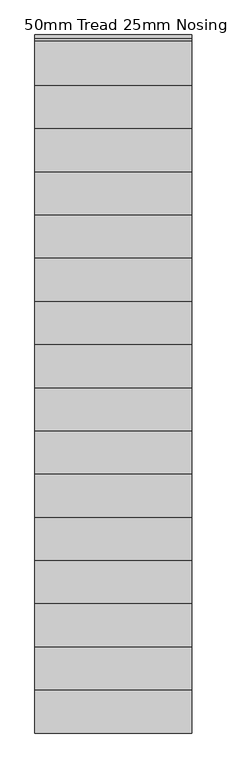
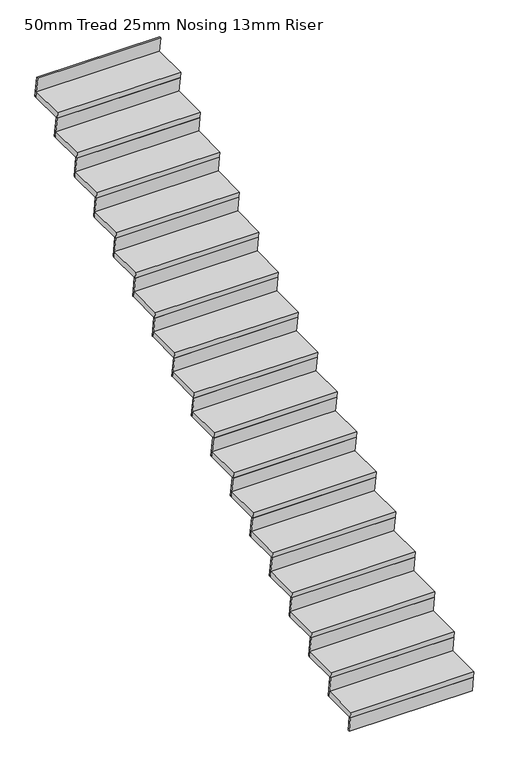
"""IFC4 building model written with IfcOpenShell, lengths in millimetres: stair flight geometry, 50mm Tread 25mm Nosing 13mm Riser."""

from ifc_helpers import new_model, si_unit, frame, origin, place, context, project, spatial, polyline, outline, extrude, source, transform, mapped, element, save


def stair_flight_50mm_tread_25mm_nosing_13mm_riser_3b40119f(model_context):
    return source(origin(), model_context, "Body", "SweptSolid", [
        extrude(outline(polyline([(-31126.6946949, 176.4705882), (-30826.6946949, 176.4705882), (-30819.6113616, 126.4705882), (-31119.6113616, 126.4705882), (-31126.6946949, 176.4705882)])), frame((121318.8827039, 0.0, 0.0), z_axis=(1.0, 0.0, 0.0), x_axis=(0.0, 1.0, 0.0)), (0.0, 0.0, 1.0), 1000.0),
        extrude(outline(polyline([(-31119.6113616, 126.4705882), (-31106.9865507, 126.4705882), (-31089.069884, 0.0), (-31101.6946949, 0.0), (-31119.6113616, 126.4705882)])), frame((121318.8827039, 0.0, 0.0), z_axis=(1.0, 0.0, 0.0), x_axis=(0.0, 1.0, 0.0)), (0.0, 0.0, 1.0), 1000.0),
        extrude(outline(polyline([(-30844.6113616, 302.9411765), (-30831.9865507, 302.9411765), (-30806.9865507, 126.4705882), (-30819.6113616, 126.4705882), (-30844.6113616, 302.9411765)])), frame((121318.8827039, 0.0, 0.0), z_axis=(1.0, 0.0, 0.0), x_axis=(0.0, 1.0, 0.0)), (0.0, 0.0, 1.0), 1000.0),
        extrude(outline(polyline([(-30851.6946949, 352.9411765), (-30551.6946949, 352.9411765), (-30544.6113616, 302.9411765), (-30844.6113616, 302.9411765), (-30851.6946949, 352.9411765)])), frame((121318.8827039, 0.0, 0.0), z_axis=(1.0, 0.0, 0.0), x_axis=(0.0, 1.0, 0.0)), (0.0, 0.0, 1.0), 1000.0),
        extrude(outline(polyline([(-30569.6113616, 479.4117647), (-30556.9865507, 479.4117647), (-30531.9865507, 302.9411765), (-30544.6113616, 302.9411765), (-30569.6113616, 479.4117647)])), frame((121318.8827039, 0.0, 0.0), z_axis=(1.0, 0.0, 0.0), x_axis=(0.0, 1.0, 0.0)), (0.0, 0.0, 1.0), 1000.0),
        extrude(outline(polyline([(-30576.6946949, 529.4117647), (-30276.6946949, 529.4117647), (-30269.6113616, 479.4117647), (-30569.6113616, 479.4117647), (-30576.6946949, 529.4117647)])), frame((121318.8827039, 0.0, 0.0), z_axis=(1.0, 0.0, 0.0), x_axis=(0.0, 1.0, 0.0)), (0.0, 0.0, 1.0), 1000.0),
        extrude(outline(polyline([(-30294.6113616, 655.8823529), (-30281.9865507, 655.8823529), (-30256.9865507, 479.4117647), (-30269.6113616, 479.4117647), (-30294.6113616, 655.8823529)])), frame((121318.8827039, 0.0, 0.0), z_axis=(1.0, 0.0, 0.0), x_axis=(0.0, 1.0, 0.0)), (0.0, 0.0, 1.0), 1000.0),
        extrude(outline(polyline([(-30301.6946949, 705.8823529), (-30001.6946949, 705.8823529), (-29994.6113616, 655.8823529), (-30294.6113616, 655.8823529), (-30301.6946949, 705.8823529)])), frame((121318.8827039, 0.0, 0.0), z_axis=(1.0, 0.0, 0.0), x_axis=(0.0, 1.0, 0.0)), (0.0, 0.0, 1.0), 1000.0),
        extrude(outline(polyline([(-30019.6113616, 832.3529412), (-30006.9865507, 832.3529412), (-29981.9865507, 655.8823529), (-29994.6113616, 655.8823529), (-30019.6113616, 832.3529412)])), frame((121318.8827039, 0.0, 0.0), z_axis=(1.0, 0.0, 0.0), x_axis=(0.0, 1.0, 0.0)), (0.0, 0.0, 1.0), 1000.0),
        extrude(outline(polyline([(-30026.6946949, 882.3529412), (-29726.6946949, 882.3529412), (-29719.6113616, 832.3529412), (-30019.6113616, 832.3529412), (-30026.6946949, 882.3529412)])), frame((121318.8827039, 0.0, 0.0), z_axis=(1.0, 0.0, 0.0), x_axis=(0.0, 1.0, 0.0)), (0.0, 0.0, 1.0), 1000.0),
        extrude(outline(polyline([(-29744.6113616, 1008.8235294), (-29731.9865507, 1008.8235294), (-29706.9865507, 832.3529412), (-29719.6113616, 832.3529412), (-29744.6113616, 1008.8235294)])), frame((121318.8827039, 0.0, 0.0), z_axis=(1.0, 0.0, 0.0), x_axis=(0.0, 1.0, 0.0)), (0.0, 0.0, 1.0), 1000.0),
        extrude(outline(polyline([(-29751.6946949, 1058.8235294), (-29451.6946949, 1058.8235294), (-29444.6113616, 1008.8235294), (-29744.6113616, 1008.8235294), (-29751.6946949, 1058.8235294)])), frame((121318.8827039, 0.0, 0.0), z_axis=(1.0, 0.0, 0.0), x_axis=(0.0, 1.0, 0.0)), (0.0, 0.0, 1.0), 1000.0),
        extrude(outline(polyline([(-29469.6113616, 1185.2941176), (-29456.9865507, 1185.2941176), (-29431.9865507, 1008.8235294), (-29444.6113616, 1008.8235294), (-29469.6113616, 1185.2941176)])), frame((121318.8827039, 0.0, 0.0), z_axis=(1.0, 0.0, 0.0), x_axis=(0.0, 1.0, 0.0)), (0.0, 0.0, 1.0), 1000.0),
        extrude(outline(polyline([(-29476.6946949, 1235.2941176), (-29176.6946949, 1235.2941176), (-29169.6113616, 1185.2941176), (-29469.6113616, 1185.2941176), (-29476.6946949, 1235.2941176)])), frame((121318.8827039, 0.0, 0.0), z_axis=(1.0, 0.0, 0.0), x_axis=(0.0, 1.0, 0.0)), (0.0, 0.0, 1.0), 1000.0),
        extrude(outline(polyline([(-29194.6113616, 1361.7647059), (-29181.9865507, 1361.7647059), (-29156.9865507, 1185.2941176), (-29169.6113616, 1185.2941176), (-29194.6113616, 1361.7647059)])), frame((121318.8827039, 0.0, 0.0), z_axis=(1.0, 0.0, 0.0), x_axis=(0.0, 1.0, 0.0)), (0.0, 0.0, 1.0), 1000.0),
        extrude(outline(polyline([(-29201.6946949, 1411.7647059), (-28901.6946949, 1411.7647059), (-28894.6113616, 1361.7647059), (-29194.6113616, 1361.7647059), (-29201.6946949, 1411.7647059)])), frame((121318.8827039, 0.0, 0.0), z_axis=(1.0, 0.0, 0.0), x_axis=(0.0, 1.0, 0.0)), (0.0, 0.0, 1.0), 1000.0),
        extrude(outline(polyline([(-28919.6113616, 1538.2352941), (-28906.9865507, 1538.2352941), (-28881.9865507, 1361.7647059), (-28894.6113616, 1361.7647059), (-28919.6113616, 1538.2352941)])), frame((121318.8827039, 0.0, 0.0), z_axis=(1.0, 0.0, 0.0), x_axis=(0.0, 1.0, 0.0)), (0.0, 0.0, 1.0), 1000.0),
        extrude(outline(polyline([(-28926.6946949, 1588.2352941), (-28626.6946949, 1588.2352941), (-28619.6113616, 1538.2352941), (-28919.6113616, 1538.2352941), (-28926.6946949, 1588.2352941)])), frame((121318.8827039, 0.0, 0.0), z_axis=(1.0, 0.0, 0.0), x_axis=(0.0, 1.0, 0.0)), (0.0, 0.0, 1.0), 1000.0),
        extrude(outline(polyline([(-28644.6113616, 1714.7058824), (-28631.9865507, 1714.7058824), (-28606.9865507, 1538.2352941), (-28619.6113616, 1538.2352941), (-28644.6113616, 1714.7058824)])), frame((121318.8827039, 0.0, 0.0), z_axis=(1.0, 0.0, 0.0), x_axis=(0.0, 1.0, 0.0)), (0.0, 0.0, 1.0), 1000.0),
        extrude(outline(polyline([(-28651.6946949, 1764.7058824), (-28351.6946949, 1764.7058824), (-28344.6113616, 1714.7058824), (-28644.6113616, 1714.7058824), (-28651.6946949, 1764.7058824)])), frame((121318.8827039, 0.0, 0.0), z_axis=(1.0, 0.0, 0.0), x_axis=(0.0, 1.0, 0.0)), (0.0, 0.0, 1.0), 1000.0),
        extrude(outline(polyline([(-28369.6113616, 1891.1764706), (-28356.9865507, 1891.1764706), (-28331.9865507, 1714.7058824), (-28344.6113616, 1714.7058824), (-28369.6113616, 1891.1764706)])), frame((121318.8827039, 0.0, 0.0), z_axis=(1.0, 0.0, 0.0), x_axis=(0.0, 1.0, 0.0)), (0.0, 0.0, 1.0), 1000.0),
        extrude(outline(polyline([(-28376.6946949, 1941.1764706), (-28076.6946949, 1941.1764706), (-28069.6113616, 1891.1764706), (-28369.6113616, 1891.1764706), (-28376.6946949, 1941.1764706)])), frame((121318.8827039, 0.0, 0.0), z_axis=(1.0, 0.0, 0.0), x_axis=(0.0, 1.0, 0.0)), (0.0, 0.0, 1.0), 1000.0),
        extrude(outline(polyline([(-28094.6113616, 2067.6470588), (-28081.9865507, 2067.6470588), (-28056.9865507, 1891.1764706), (-28069.6113616, 1891.1764706), (-28094.6113616, 2067.6470588)])), frame((121318.8827039, 0.0, 0.0), z_axis=(1.0, 0.0, 0.0), x_axis=(0.0, 1.0, 0.0)), (0.0, 0.0, 1.0), 1000.0),
        extrude(outline(polyline([(-28101.6946949, 2117.6470588), (-27801.6946949, 2117.6470588), (-27794.6113616, 2067.6470588), (-28094.6113616, 2067.6470588), (-28101.6946949, 2117.6470588)])), frame((121318.8827039, 0.0, 0.0), z_axis=(1.0, 0.0, 0.0), x_axis=(0.0, 1.0, 0.0)), (0.0, 0.0, 1.0), 1000.0),
        extrude(outline(polyline([(-27819.6113616, 2244.1176471), (-27806.9865507, 2244.1176471), (-27781.9865507, 2067.6470588), (-27794.6113616, 2067.6470588), (-27819.6113616, 2244.1176471)])), frame((121318.8827039, 0.0, 0.0), z_axis=(1.0, 0.0, 0.0), x_axis=(0.0, 1.0, 0.0)), (0.0, 0.0, 1.0), 1000.0),
        extrude(outline(polyline([(-27826.6946949, 2294.1176471), (-27526.6946949, 2294.1176471), (-27519.6113616, 2244.1176471), (-27819.6113616, 2244.1176471), (-27826.6946949, 2294.1176471)])), frame((121318.8827039, 0.0, 0.0), z_axis=(1.0, 0.0, 0.0), x_axis=(0.0, 1.0, 0.0)), (0.0, 0.0, 1.0), 1000.0),
        extrude(outline(polyline([(-27544.6113616, 2420.5882353), (-27531.9865507, 2420.5882353), (-27506.9865507, 2244.1176471), (-27519.6113616, 2244.1176471), (-27544.6113616, 2420.5882353)])), frame((121318.8827039, 0.0, 0.0), z_axis=(1.0, 0.0, 0.0), x_axis=(0.0, 1.0, 0.0)), (0.0, 0.0, 1.0), 1000.0),
        extrude(outline(polyline([(-27551.6946949, 2470.5882353), (-27251.6946949, 2470.5882353), (-27244.6113616, 2420.5882353), (-27544.6113616, 2420.5882353), (-27551.6946949, 2470.5882353)])), frame((121318.8827039, 0.0, 0.0), z_axis=(1.0, 0.0, 0.0), x_axis=(0.0, 1.0, 0.0)), (0.0, 0.0, 1.0), 1000.0),
        extrude(outline(polyline([(-27269.6113616, 2597.0588235), (-27256.9865507, 2597.0588235), (-27231.9865507, 2420.5882353), (-27244.6113616, 2420.5882353), (-27269.6113616, 2597.0588235)])), frame((121318.8827039, 0.0, 0.0), z_axis=(1.0, 0.0, 0.0), x_axis=(0.0, 1.0, 0.0)), (0.0, 0.0, 1.0), 1000.0),
        extrude(outline(polyline([(-27276.6946949, 2647.0588235), (-26976.6946949, 2647.0588235), (-26969.6113616, 2597.0588235), (-27269.6113616, 2597.0588235), (-27276.6946949, 2647.0588235)])), frame((121318.8827039, 0.0, 0.0), z_axis=(1.0, 0.0, 0.0), x_axis=(0.0, 1.0, 0.0)), (0.0, 0.0, 1.0), 1000.0),
        extrude(outline(polyline([(-26994.6113616, 2773.5294118), (-26981.9865507, 2773.5294118), (-26956.9865507, 2597.0588235), (-26969.6113616, 2597.0588235), (-26994.6113616, 2773.5294118)])), frame((121318.8827039, 0.0, 0.0), z_axis=(1.0, 0.0, 0.0), x_axis=(0.0, 1.0, 0.0)), (0.0, 0.0, 1.0), 1000.0),
        extrude(outline(polyline([(-26719.6113616, 2950.0), (-26706.9865507, 2950.0), (-26681.9865507, 2773.5294118), (-26694.6113616, 2773.5294118), (-26719.6113616, 2950.0)])), frame((121318.8827039, 0.0, 0.0), z_axis=(1.0, 0.0, 0.0), x_axis=(0.0, 1.0, 0.0)), (0.0, 0.0, 1.0), 1000.0),
        extrude(outline(polyline([(-27001.6946949, 2823.5294118), (-26701.6946949, 2823.5294118), (-26694.6113616, 2773.5294118), (-26994.6113616, 2773.5294118), (-27001.6946949, 2823.5294118)])), frame((121318.8827039, 0.0, 0.0), z_axis=(1.0, 0.0, 0.0), x_axis=(0.0, 1.0, 0.0)), (0.0, 0.0, 1.0), 1000.0),
    ])


if __name__ == "__main__":
    model = new_model("IFC4")
    model_context = context("Model", 3, world=origin())
    ifc_project = project(units=[si_unit("LENGTHUNIT", "METRE", prefix="MILLI")], contexts=[model_context])
    site = spatial("IfcSite", under=ifc_project)
    building = spatial("IfcBuilding", under=site)
    placement = place(None, origin())
    stair_flight_50mm_tread_25mm_nosing_13mm_riser_shape = stair_flight_50mm_tread_25mm_nosing_13mm_riser_3b40119f(model_context)
    element("IfcStairFlight", 1, ObjectType="50mm Tread 25mm Nosing 13mm Riser", at=placement, inside=building, context=model_context, shape_type="MappedRepresentation", body=[
        mapped(stair_flight_50mm_tread_25mm_nosing_13mm_riser_shape, transform((0.0, 0.0, 0.0), x_axis=(1.0, 0.0, 0.0), y_axis=(0.0, 1.0, 0.0), z_axis=(0.0, 0.0, 1.0))),
    ])
    save(model, "model.ifc")
